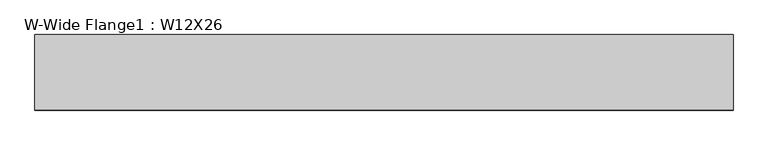
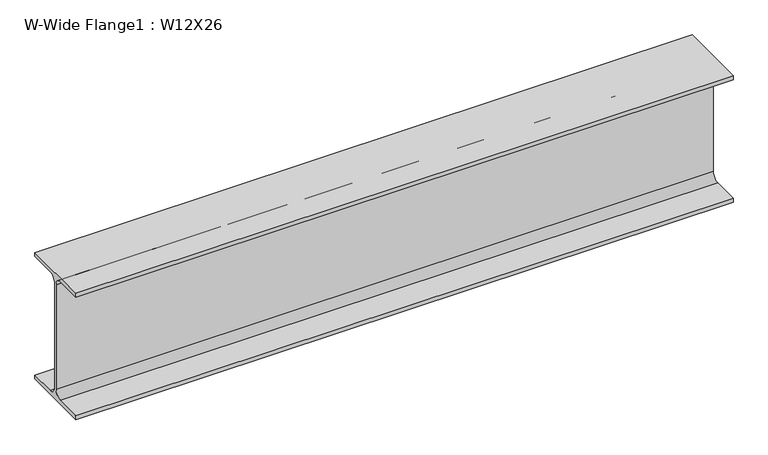
"""IFC4 building model written with IfcOpenShell, lengths in millimetres: beam geometry, W-Wide Flange1 : W12X26."""

from ifc_helpers import new_model, si_unit, point, frame, frame_2d, origin, place, context, project, spatial, polyline, circle_curve, trimmed, segment, composite_curve, outline, extrude, source, transform, mapped, element, save


def w_wide_flange1_w12x26_1c87423a(model_context):
    return source(origin(), model_context, "Body", "SweptSolid", [
        extrude(outline(composite_curve([segment(polyline([(82.423, -145.288), (82.423, -154.94), (-82.423, -154.94), (-82.423, -145.288), (-20.2565, -145.288)]), True, "CONTINUOUS"), segment(trimmed(circle_curve(frame_2d((-20.2565, -127.9525)), 17.3355), [point((-20.2565, -145.288))], [point((-2.921, -127.9525))], True, "CARTESIAN"), True, "CONTINUOUS"), segment(polyline([(-2.921, -127.9525), (-2.921, 127.9525)]), True, "CONTINUOUS"), segment(trimmed(circle_curve(frame_2d((-20.2565, 127.9525)), 17.3355), [point((-2.921, 127.9525))], [point((-20.2565, 145.288))], True, "CARTESIAN"), True, "CONTINUOUS"), segment(polyline([(-20.2565, 145.288), (-82.423, 145.288), (-82.423, 154.94), (82.423, 154.94), (82.423, 145.288), (20.2565, 145.288)]), True, "CONTINUOUS"), segment(trimmed(circle_curve(frame_2d((20.2565, 127.9525)), 17.3355), [point((20.2565, 145.288))], [point((2.921, 127.9525))], True, "CARTESIAN"), True, "CONTINUOUS"), segment(polyline([(2.921, 127.9525), (2.921, -127.9525)]), True, "CONTINUOUS"), segment(trimmed(circle_curve(frame_2d((20.2565, -127.9525)), 17.3355), [point((2.921, -127.9525))], [point((20.2565, -145.288))], True, "CARTESIAN"), True, "CONTINUOUS"), segment(polyline([(20.2565, -145.288), (82.423, -145.288)]), True, "CONTINUOUS")], self_intersect=False)), frame((-741.532309, 0.0, 0.0), z_axis=(1.0, 0.0, 0.0), x_axis=(0.0, 1.0, 0.0)), (0.0, 0.0, 1.0), 1522.8264389),
    ])


if __name__ == "__main__":
    model = new_model("IFC4")
    model_context = context("Model", 3, world=origin())
    ifc_project = project(units=[si_unit("LENGTHUNIT", "METRE", prefix="MILLI")], contexts=[model_context])
    site = spatial("IfcSite", under=ifc_project)
    building = spatial("IfcBuilding", under=site)
    placement = place(None, origin())
    w_wide_flange1_w12x26_shape = w_wide_flange1_w12x26_1c87423a(model_context)
    element("IfcBeam", 1, ObjectType="W-Wide Flange1 : W12X26", at=placement, inside=building, context=model_context, shape_type="MappedRepresentation", body=[
        mapped(w_wide_flange1_w12x26_shape, transform((0.0, 0.0, 0.0), x_axis=(1.0, 0.0, 0.0), y_axis=(0.0, 1.0, 0.0), z_axis=(0.0, 0.0, 1.0))),
    ])
    save(model, "model.ifc")

# Revit data of these elements
# Type "W-Wide Flange1 : W12X26"
#   Assembly Code = "B10"
#   W = 26
#   Start Extension Calculation [instance default] = 10' - 0"
#   Start Extension [instance default] = -0' - 0 1/2"
#   End Extension Calculation [instance default] = 10' - 0"
#   End Extension [instance default] = -0' - 0 1/2"
#   Length [instance default] = 5' - 0"
#   bf = 0' - 6.49"
#   d = 1' - 0.2"
#   k = 0' - 1 1/16"
#   k2 = 0' - 0.6825"
#   tf = 0' - 0.38"
#   tw = 0' - 0.23"
#   A = 0.053125 SF
#   Structural Material [instance default] = Metal - Steel - ASTM A992
# Element 1 (IfcBeam, "W-Wide Flange1 : W12X26")
#   Materials on its faces: "Metal - Steel - ASTM A992"
# Materials
#   "Metal - Steel - ASTM A992": class "Metal", colour RGB 199 199 199, transparency 0
